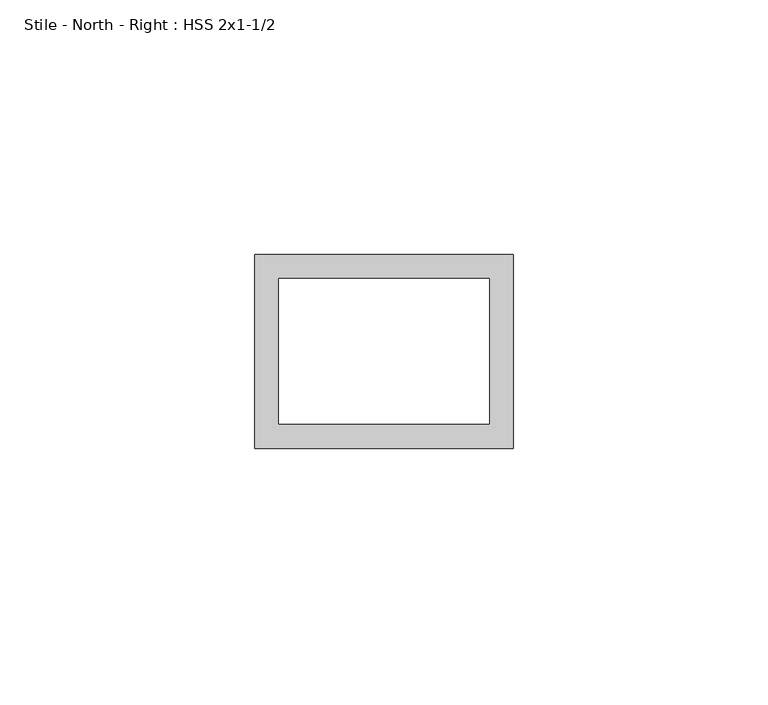
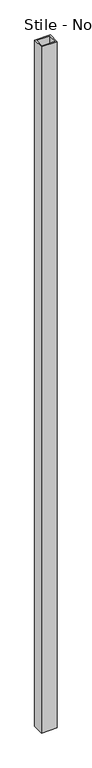
"""IFC4 building model written with IfcOpenShell, lengths in millimetres: proxy geometry, Stile - North - Right : HSS 2x1-1/2."""

from ifc_helpers import new_model, si_unit, frame, origin, place, context, project, spatial, polyline, outline, extrude, source, transform, mapped, element, save


def stile_north_right_hss_2x1_1_2_44639784(model_context):
    return source(origin(), model_context, "Body", "SweptSolid", [
        extrude(outline(polyline([(587365.8934739, -532839.3663841), (587416.6934739, -532839.3663841), (587416.6934739, -532877.4663841), (587365.8934739, -532877.4663841), (587365.8934739, -532839.3663841)]), holes=[polyline([(587370.6559739, -532844.1288841), (587370.6559739, -532872.7038841), (587411.9309739, -532872.7038841), (587411.9309739, -532844.1288841), (587370.6559739, -532844.1288841)])]), frame((0.0, 0.0, 50.8), z_axis=(0.0, 0.0, 1.0), x_axis=(1.0, 0.0, 0.0)), (0.0, 0.0, 1.0), 2349.5),
    ])


if __name__ == "__main__":
    model = new_model("IFC4")
    model_context = context("Model", 3, world=origin())
    ifc_project = project(units=[si_unit("LENGTHUNIT", "METRE", prefix="MILLI")], contexts=[model_context])
    site = spatial("IfcSite", under=ifc_project)
    building = spatial("IfcBuilding", under=site)
    placement = place(None, origin())
    stile_north_right_hss_2x1_1_2_shape = stile_north_right_hss_2x1_1_2_44639784(model_context)
    element("IfcBuildingElementProxy", 1, Name="Stile - North - Right : HSS 2x1-1/2", ObjectType="Stile - North - Right : HSS 2x1-1/2", at=placement, inside=building, context=model_context, shape_type="MappedRepresentation", body=[
        mapped(stile_north_right_hss_2x1_1_2_shape, transform((0.0, 0.0, 0.0), x_axis=(1.0, 0.0, 0.0), y_axis=(0.0, 1.0, 0.0), z_axis=(0.0, 0.0, 1.0))),
    ])
    save(model, "model.ifc")

# Revit data of these elements
# Element 1 (IfcBuildingElementProxy, "Stile - North - Right : HSS 2x1-1/2")
#   Materials on its faces: "1-1/2\"X2\" GALV. STL HSS TUBING"
# Materials
#   "1-1/2\"X2\" GALV. STL HSS TUBING": class "Generic", colour RGB 211 211 207, transparency 0, Cost = 0
